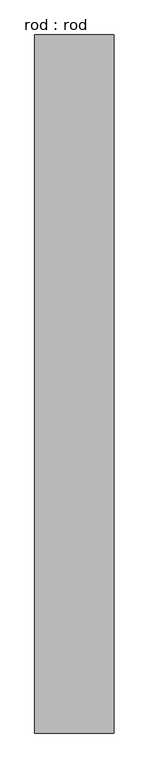
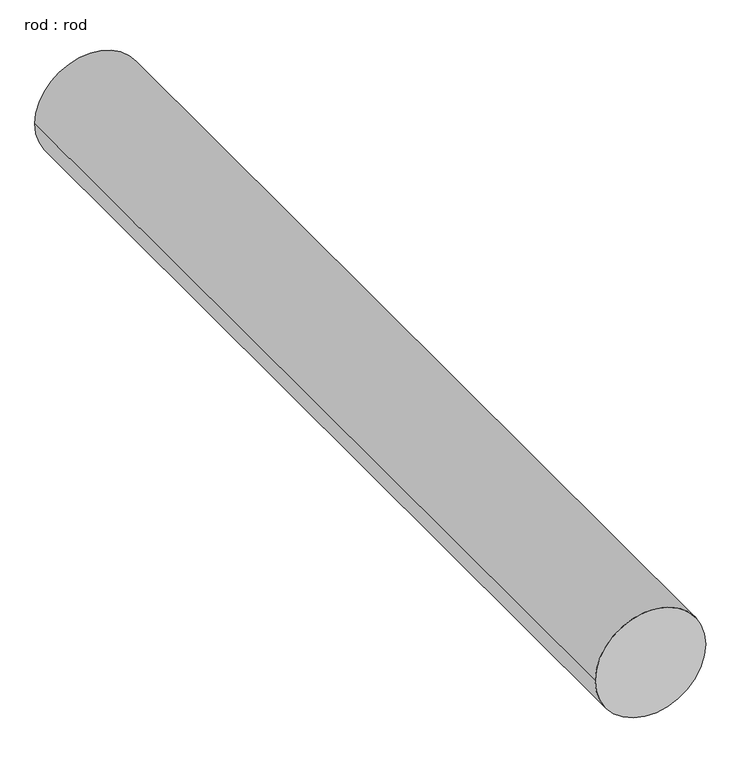
"""IFC4 building model written with IfcOpenShell, lengths in millimetres: proxy geometry, rod : rod."""

from ifc_helpers import new_model, si_unit, point, frame, frame_2d, origin, place, context, project, spatial, circle_curve, trimmed, segment, composite_curve, outline, extrude, source, transform, mapped, element, save


def rod_rod_011496a8(model_context):
    return source(origin(), model_context, "Body", "SweptSolid", [
        extrude(outline(composite_curve([segment(trimmed(circle_curve(frame_2d((0.0108462, 0.0)), 200.0), [point((0.0108462, 200.0))], [point((0.0108462, -200.0))], False, "CARTESIAN"), True, "CONTINUOUS"), segment(trimmed(circle_curve(frame_2d((0.0108462, 0.0)), 200.0), [point((0.0108462, -200.0))], [point((0.0108462, 200.0))], False, "CARTESIAN"), True, "CONTINUOUS")], self_intersect=False)), frame((0.0, 2335.5857582, 0.0), z_axis=(0.0, 1.0, 0.0), x_axis=(0.0, 0.0, 1.0)), (0.0, 0.0, 1.0), 3514.2857143),
    ])


if __name__ == "__main__":
    model = new_model("IFC4")
    model_context = context("Model", 3, world=origin())
    ifc_project = project(units=[si_unit("LENGTHUNIT", "METRE", prefix="MILLI")], contexts=[model_context])
    site = spatial("IfcSite", under=ifc_project)
    building = spatial("IfcBuilding", under=site)
    placement = place(None, origin())
    rod_rod_shape = rod_rod_011496a8(model_context)
    element("IfcBuildingElementProxy", 1, Name="rod : rod", ObjectType="rod : rod", at=placement, inside=building, context=model_context, shape_type="MappedRepresentation", body=[
        mapped(rod_rod_shape, transform((0.0, 0.0, 0.0), x_axis=(1.0, 0.0, 0.0), y_axis=(0.0, 1.0, 0.0), z_axis=(0.0, 0.0, 1.0))),
    ])
    save(model, "model.ifc")

# Revit data of these elements
# Project information
#   Project Issue Date = "Issue Date"
#   Project Status = "Project Status"
#   Client Name = "Owner"
#   Project Address = "Enter address here"
#   Project Name = "Project Name"
#   Project Number = "0001"
# Type "rod : rod"
#   Default Elevation = 0
